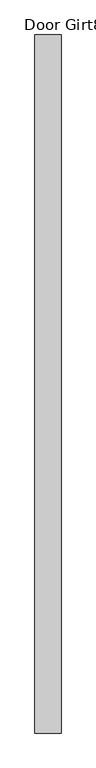
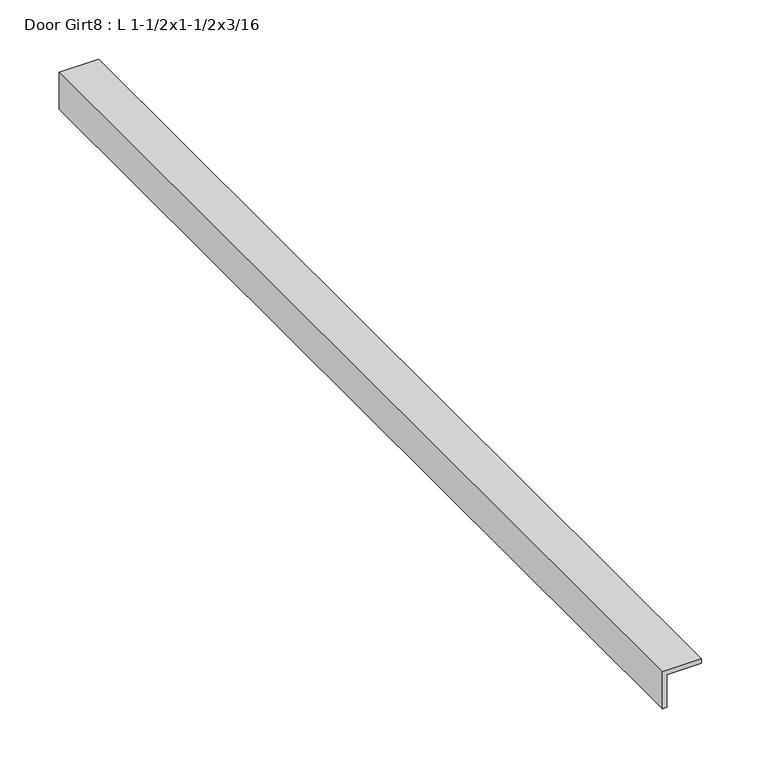
"""IFC4 building model written with IfcOpenShell, lengths in millimetres: proxy geometry, Door Girt8 : L 1-1/2x1-1/2x3/16."""

from ifc_helpers import new_model, si_unit, frame, origin, place, context, project, spatial, polyline, outline, extrude, source, transform, mapped, element, save


def door_girt8_l_1_1_2x1_1_2x3_16_602a1831(model_context):
    return source(origin(), model_context, "Body", "SweptSolid", [
        extrude(outline(polyline([(1625.6, 587403.9934739), (1625.6, 587365.8934739), (1587.5, 587365.8934739), (1587.5, 587370.6559739), (1620.8375, 587370.6559739), (1620.8375, 587403.9934739), (1625.6, 587403.9934739)])), frame((0.0, -533937.9163841, 0.0), z_axis=(0.0, 1.0, 0.0), x_axis=(0.0, 0.0, 1.0)), (0.0, 0.0, 1.0), 1016.0),
    ])


if __name__ == "__main__":
    model = new_model("IFC4")
    model_context = context("Model", 3, world=origin())
    ifc_project = project(units=[si_unit("LENGTHUNIT", "METRE", prefix="MILLI")], contexts=[model_context])
    site = spatial("IfcSite", under=ifc_project)
    building = spatial("IfcBuilding", under=site)
    placement = place(None, origin())
    door_girt8_l_1_1_2x1_1_2x3_16_shape = door_girt8_l_1_1_2x1_1_2x3_16_602a1831(model_context)
    element("IfcBuildingElementProxy", 1, Name="Door Girt8 : L 1-1/2x1-1/2x3/16", ObjectType="Door Girt8 : L 1-1/2x1-1/2x3/16", at=placement, inside=building, context=model_context, shape_type="MappedRepresentation", body=[
        mapped(door_girt8_l_1_1_2x1_1_2x3_16_shape, transform((0.0, 0.0, 0.0), x_axis=(1.0, 0.0, 0.0), y_axis=(0.0, 1.0, 0.0), z_axis=(0.0, 0.0, 1.0))),
    ])
    save(model, "model.ifc")

# Revit data of these elements
# Element 1 (IfcBuildingElementProxy, "Door Girt8 : L 1-1/2x1-1/2x3/16")
#   Materials on its faces: "1-1/2\"X1-1/2\" GALV. STL L"
# Materials
#   "1-1/2\"X1-1/2\" GALV. STL L": class "Generic", colour RGB 211 211 207, transparency 0, Cost = 0
